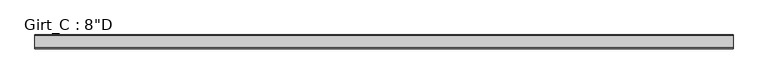
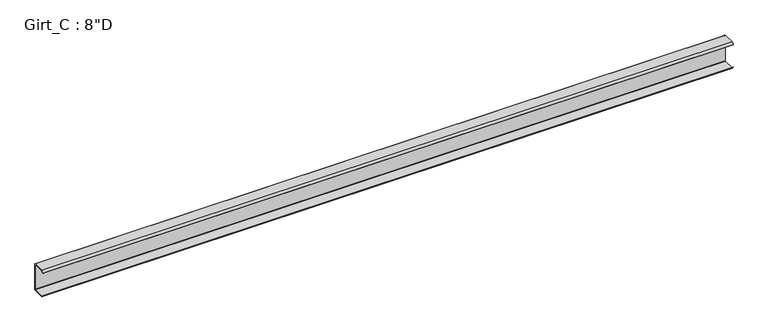
"""IFC4 building model written with IfcOpenShell, lengths in millimetres: beam geometry."""

from ifc_helpers import new_model, si_unit, point, frame, frame_2d, origin, place, context, project, spatial, polyline, circle_curve, trimmed, segment, composite_curve, outline, extrude, source, transform, mapped, element, save


def beam_0a0f1977(model_context):
    return source(origin(), model_context, "Body", "SweptSolid", [
        extrude(outline(composite_curve([segment(polyline([(-87.5109375, 101.6), (-3.3734375, 101.6)]), True, "CONTINUOUS"), segment(trimmed(circle_curve(frame_2d((-3.3734375, 96.8375)), 4.7625), [point((-3.3734375, 101.6))], [point((1.3890625, 96.8375))], False, "CARTESIAN"), True, "CONTINUOUS"), segment(polyline([(1.3890625, 96.8375), (1.3890625, -96.8375)]), True, "CONTINUOUS"), segment(trimmed(circle_curve(frame_2d((-3.3734375, -96.8375)), 4.7625), [point((1.3890625, -96.8375))], [point((-3.3734375, -101.6))], False, "CARTESIAN"), True, "CONTINUOUS"), segment(polyline([(-3.3734375, -101.6), (-87.5109375, -101.6), (-99.7792647, -86.979177), (-97.6510975, -85.1934327), (-86.2154765, -98.821875), (-3.2694106, -98.821875)]), True, "CONTINUOUS"), segment(trimmed(circle_curve(frame_2d((-3.3748024, -96.8389339)), 1.9857399), [point((-3.2694106, -98.821875))], [point((-1.3890625, -96.8389339))], True, "CARTESIAN"), True, "CONTINUOUS"), segment(polyline([(-1.3890625, -96.8389339), (-1.3890625, 96.8381931)]), True, "CONTINUOUS"), segment(trimmed(circle_curve(frame_2d((-3.3741066, 96.8381931)), 1.9850441), [point((-1.3890625, 96.8381931))], [point((-3.3005807, 98.821875))], True, "CARTESIAN"), True, "CONTINUOUS"), segment(polyline([(-3.3005807, 98.821875), (-86.2154765, 98.821875), (-97.6278742, 85.221109), (-99.7560415, 87.0068534), (-87.5109375, 101.6)]), True, "CONTINUOUS")], self_intersect=False)), frame((-2543.96875, 0.0, 0.0), z_axis=(1.0, 0.0, 0.0), x_axis=(0.0, 1.0, 0.0)), (0.0, 0.0, 1.0), 5015.8015),
    ])


if __name__ == "__main__":
    model = new_model("IFC4")
    model_context = context("Model", 3, world=origin())
    ifc_project = project(units=[si_unit("LENGTHUNIT", "METRE", prefix="MILLI")], contexts=[model_context])
    site = spatial("IfcSite", under=ifc_project)
    building = spatial("IfcBuilding", under=site)
    placement = place(None, origin())
    beam_shape = beam_0a0f1977(model_context)
    element("IfcBeam", 1, ObjectType="Girt_C : 8\"D", at=placement, inside=building, context=model_context, shape_type="MappedRepresentation", body=[
        mapped(beam_shape, transform((0.0, 0.0, 0.0), x_axis=(1.0, 0.0, 0.0), y_axis=(0.0, 1.0, 0.0), z_axis=(0.0, 0.0, 1.0))),
    ])
    save(model, "model.ifc")

# Revit data of these elements
# Type "Girt_C : 8\"D"
#   half leg = 0' - 1 3/4"
#   Web_Thickness = 0' - 0 7/64"
#   Length [instance default] = 10' - 0"
#   Leg_1 = 0' - 3 1/2"
#   Height = 0' - 8"
#   Structural Material [instance default] = none
# Element 1 (IfcBeam, "Girt_C : 8\"D")
#   Structural Material = CEE' SECTION (8.0x3.5C - SEE STRUCT. DWGS)
#   Materials on its faces: "CEE' SECTION (8.0x3.5C - SEE STRUCT. DWGS)"
# Materials
#   "CEE' SECTION (8.0x3.5C - SEE STRUCT. DWGS)": class "Metal", colour RGB 137 146 153, transparency 0, Description = "Steel, mill finish", Cost = 0
